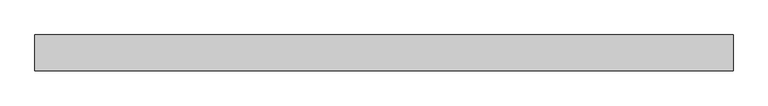
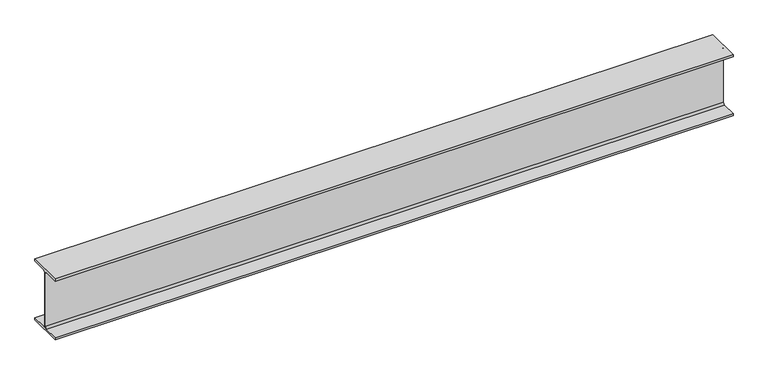
"""IFC4 building model written with IfcOpenShell, lengths in millimetres: beam geometry, Old_Steel Beam_H-KSD3502 : H_SB_ASB_H-200×200x8x12."""

from ifc_helpers import new_model, si_unit, point, frame, frame_2d, origin, place, context, project, spatial, polyline, circle_curve, trimmed, segment, composite_curve, outline, extrude, source, transform, mapped, element, save


def beam_35ee4ea3(model_context):
    return source(origin(), model_context, "Body", "SweptSolid", [
        extrude(outline(composite_curve([segment(polyline([(82.5, -141.5), (82.5, -151.7), (-82.5, -151.7), (-82.5, -141.5), (-11.9, -141.5)]), True, "CONTINUOUS"), segment(trimmed(circle_curve(frame_2d((-11.9, -132.6)), 8.9), [point((-11.9, -141.5))], [point((-3.0, -132.6))], True, "CARTESIAN"), True, "CONTINUOUS"), segment(polyline([(-3.0, -132.6), (-3.0, 132.6)]), True, "CONTINUOUS"), segment(trimmed(circle_curve(frame_2d((-11.9, 132.6)), 8.9), [point((-3.0, 132.6))], [point((-11.9, 141.5))], True, "CARTESIAN"), True, "CONTINUOUS"), segment(polyline([(-11.9, 141.5), (-82.5, 141.5), (-82.5, 151.7), (82.5, 151.7), (82.5, 141.5), (11.9, 141.5)]), True, "CONTINUOUS"), segment(trimmed(circle_curve(frame_2d((11.9, 132.6)), 8.9), [point((11.9, 141.5))], [point((3.0, 132.6))], True, "CARTESIAN"), True, "CONTINUOUS"), segment(polyline([(3.0, 132.6), (3.0, -132.6)]), True, "CONTINUOUS"), segment(trimmed(circle_curve(frame_2d((11.9, -132.6)), 8.9), [point((3.0, -132.6))], [point((11.9, -141.5))], True, "CARTESIAN"), True, "CONTINUOUS"), segment(polyline([(11.9, -141.5), (82.5, -141.5)]), True, "CONTINUOUS")], self_intersect=False)), frame((-1481.293912, 0.0, 0.0), z_axis=(1.0, 0.0, 0.0), x_axis=(0.0, 1.0, 0.0)), (0.0, 0.0, 1.0), 3203.0379922),
    ])


if __name__ == "__main__":
    model = new_model("IFC4")
    model_context = context("Model", 3, world=origin())
    ifc_project = project(units=[si_unit("LENGTHUNIT", "METRE", prefix="MILLI")], contexts=[model_context])
    site = spatial("IfcSite", under=ifc_project)
    building = spatial("IfcBuilding", under=site)
    placement = place(None, origin())
    beam_shape = beam_35ee4ea3(model_context)
    element("IfcBeam", 1, ObjectType="Old_Steel Beam_H-KSD3502 : H_SB_ASB_H-200×200x8x12", at=placement, inside=building, context=model_context, shape_type="MappedRepresentation", body=[
        mapped(beam_shape, transform((0.0, 0.0, 0.0), x_axis=(1.0, 0.0, 0.0), y_axis=(0.0, 1.0, 0.0), z_axis=(0.0, 0.0, 1.0))),
    ])
    save(model, "model.ifc")

# Revit data of these elements
# Type "Old_Steel Beam_H-KSD3502 : H_SB_ASB_H-200×200x8x12"
#   Width = 20.0 cm
#   Web Thickness = 0.8 cm
#   Web Fillet = 1.3 cm
#   Warping Constant = 141376.0 cm⁶
#   Torsional Moment of Inertia = 26.2485 cm⁴
#   Torsional Modulus = 1.0 cm³
#   Section Area = 63.53 cm²
#   Plastic Modulus weak axis = 244.0 cm³
#   Plastic Modulus strong axis = 525.0 cm³
#   Perimeter = 1.16 m²/m
#   Nominal Weight = 49.90 kgf/m
#   Moment of Inertia weak axis = 1600.00 cm⁴
#   Moment of Inertia strong axis = 4720.00 cm⁴
#   Height = 20.0 cm
#   Flange Thickness = 1.2 cm
#   Elastic Modulus weak axis = 160.0 cm³
#   Elastic Modulus strong axis = 472.0 cm³
#   Centroid Vertical = 10.0 cm
#   Centroid Horizontal = 10.0 cm
#   Length [instance default] = 1.5240 m
#   Structural Material [instance default] = Steel, 45-345
#   Assembly Code = ""
# Element 1 (IfcBeam, "Old_Steel Beam_H-KSD3502 : H_SB_ASB_H-200×200x8x12")
#   Structural Material = none
# Materials
#   "Steel, 45-345": class "Metal", colour RGB 189 187 185, transparency 0, Description = "Steel 345 MPa", Cost = 0
